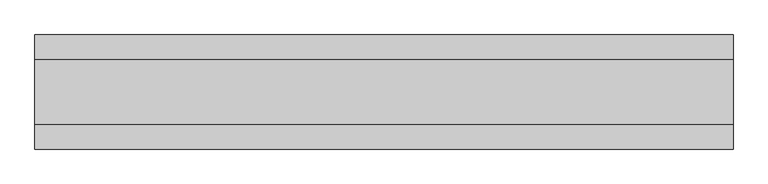
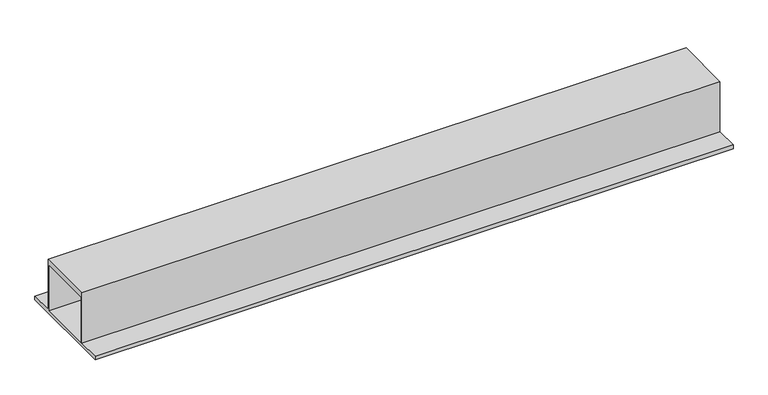
"""IFC4 building model written with IfcOpenShell, lengths in millimetres: beam geometry, NLRS_28_SF_LIB_stalen ligger THQ-AV-CWV-MMBS-SRP_gen_rsf : stalen ligger_gen__THQ_280x10-290x30-550x20."""

from ifc_helpers import new_model, si_unit, frame, origin, place, context, project, spatial, polyline, outline, extrude, source, transform, mapped, element, save


def beam_87fc56b5(model_context):
    return source(origin(), model_context, "Body", "SweptSolid", [
        extrude(outline(polyline([(143.5, 280.0), (143.5, 0.0), (263.5, 0.0), (263.5, -20.0), (-286.5, -20.0), (-286.5, 0.0), (-166.5, 0.0), (-166.5, 280.0), (143.5, 280.0)]), holes=[polyline([(133.5, 0.0), (133.5, 250.0), (-156.5, 250.0), (-156.5, 0.0), (133.5, 0.0)])]), frame((-1812.5, 0.0, 0.0), z_axis=(1.0, 0.0, 0.0), x_axis=(0.0, 1.0, 0.0)), (0.0, 0.0, 1.0), 3365.0),
    ])


if __name__ == "__main__":
    model = new_model("IFC4")
    model_context = context("Model", 3, world=origin())
    ifc_project = project(units=[si_unit("LENGTHUNIT", "METRE", prefix="MILLI")], contexts=[model_context])
    site = spatial("IfcSite", under=ifc_project)
    building = spatial("IfcBuilding", under=site)
    placement = place(None, origin())
    beam_shape = beam_87fc56b5(model_context)
    element("IfcBeam", 1, ObjectType="NLRS_28_SF_LIB_stalen ligger THQ-AV-CWV-MMBS-SRP_gen_rsf : stalen ligger_gen__THQ_280x10-290x30-550x20", at=placement, inside=building, context=model_context, shape_type="MappedRepresentation", body=[
        mapped(beam_shape, transform((0.0, 0.0, 0.0), x_axis=(1.0, 0.0, 0.0), y_axis=(0.0, 1.0, 0.0), z_axis=(0.0, 0.0, 1.0))),
    ])
    save(model, "model.ifc")

# Revit data of these elements
# Type "NLRS_28_SF_LIB_stalen ligger THQ-AV-CWV-MMBS-SRP_gen_rsf : stalen ligger_gen__THQ_280x10-290x30-550x20"
#   Type IfcGUID = "2GRbcre991teoKeCLB8MAm"
#   IfcExportAs = "IfcBeamType"
#   Type Comments = "THQ 280x10-290x30-550x20"
#   Model = " "
#   Manufacturer = " "
#   Fire Rating = " "
#   Description = "stalen ligger THQ 280x10-290x30-550x20"
#   Assembly Code = "28.11"
#   tw = 10 mm
#   tu = 20 mm
#   to = 30 mm
#   h = 280 mm
#   bu = 550 mm
#   bo = 290 mm
#   NLRS_C_lengte [instance default] = 1500 mm
#   Length [instance default] = 1500 mm
#   RSF_C_vullen_met_beton [instance default] = no
#   RSF_C_petligger = no
#   RSF_C_hoedligger = yes
#   Structural Material = NLRS_h2_staal_gen_rsf
#   Keynote = ""
# Element 1 (IfcBeam, "NLRS_28_SF_LIB_stalen ligger THQ-AV-CWV-MMBS-SRP_gen_rsf : stalen ligger_gen__THQ_280x10-290x30-550x20")
#   NLRS_C_lengte = 3625 mm
#   Materials on its faces: "NLRS_h2_staal_gen_rsf"
# Materials
#   "NLRS_h2_staal_gen_rsf": class "H - Metaal", colour RGB 189 187 185, transparency 0, Keynote = "h2", Manufacturer = "Revit Standards Foundation", URL = "www.revitstandards.org", Description = "staal", Cost = 0
